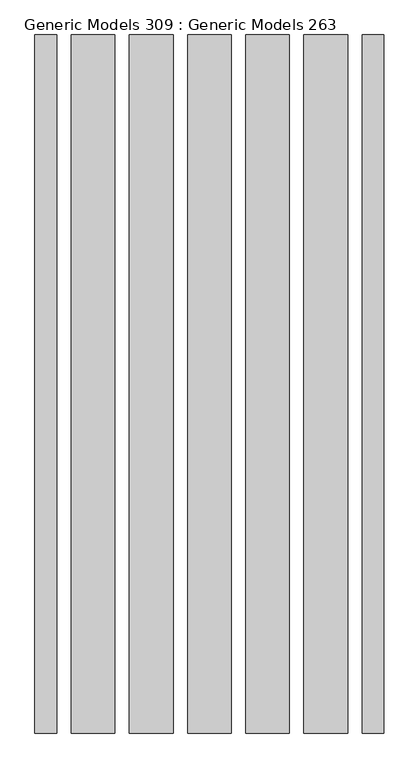
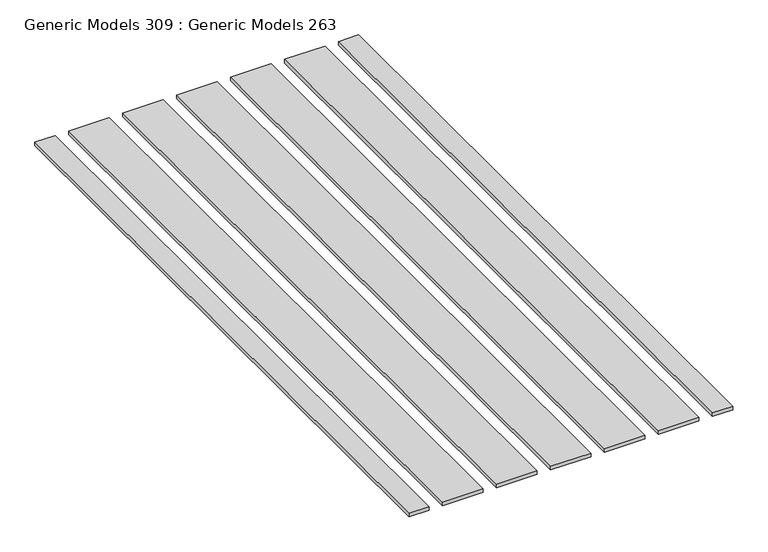
"""IFC4 building model written with IfcOpenShell, lengths in millimetres: proxy geometry, Generic Models 309 : Generic Models 263."""

import ifcopenshell
import ifcopenshell.guid

model = None  # the IFC model being written
_history = None  # IfcOwnerHistory: only IFC2X3 demands one
_inside = {}  # id of a spatial element -> (the spatial element, [elements in it])
_under = {}  # id of a project, library or spatial element -> (it, [spatial elements below it])
_declared = {}  # id of a project -> (the project, [libraries it declares])
_typed = {}  # id of a type object -> (the type object, [elements of that type])
_made_of = {}  # id of a material, layer set ... -> (it, [elements and type objects made of it])


def new_model(schema):
    """Start an empty IFC model of exactly this schema.

    Asked for "IFC4X3", IfcOpenShell would pick the latest addendum, in which some entities
    have other attributes; the version numbers below select the first issue.
    IFC2X3 requires an IfcOwnerHistory on every rooted entity: one is made here for all.
    """
    global model, _history
    if schema == "IFC4X3":
        model = ifcopenshell.file(schema_version=(4, 3, 0, 0))
    else:
        model = ifcopenshell.file(schema=schema)
    _inside.clear()
    _under.clear()
    _declared.clear()
    _typed.clear()
    _made_of.clear()
    _history = None
    if model.schema == "IFC2X3":
        org = make("IfcOrganization", Name="unknown")
        user = make(
            "IfcPersonAndOrganization",
            ThePerson=make("IfcPerson", FamilyName="unknown"),
            TheOrganization=org,
        )
        app = make(
            "IfcApplication",
            ApplicationDeveloper=org,
            Version="unknown",
            ApplicationFullName="unknown",
            ApplicationIdentifier="unknown",
        )
        _history = make(
            "IfcOwnerHistory",
            OwningUser=user,
            OwningApplication=app,
            ChangeAction="ADDED",
            CreationDate=0,
        )
    return model


def make(cls, **values):
    """One entity of the class cls with the attributes given. An attribute that is None is left unset."""
    return model.create_entity(
        cls, **{name: value for name, value in values.items() if value is not None}
    )


def rooted(cls, **values):
    """An entity with a GlobalId (a new one), such as an element, a storey or a relation."""
    return make(cls, GlobalId=ifcopenshell.guid.new(), OwnerHistory=_history, **values)


def si_unit(unit_type, name, prefix=None):
    """IfcSIUnit, for example si_unit("LENGTHUNIT", "METRE", prefix="MILLI")."""
    return make("IfcSIUnit", UnitType=unit_type, Prefix=prefix, Name=name)


def assignment(units):
    """IfcUnitAssignment: the units of a project."""
    return None if units is None else make("IfcUnitAssignment", Units=units)


def point(xyz):
    """IfcCartesianPoint."""
    return None if xyz is None else make("IfcCartesianPoint", Coordinates=xyz)


def direction(xyz):
    """IfcDirection."""
    return None if xyz is None else make("IfcDirection", DirectionRatios=xyz)


def frame(location, z_axis=None, x_axis=None):
    """IfcAxis2Placement3D, a coordinate frame: its origin and axes. An axis left out is left unset."""
    return make(
        "IfcAxis2Placement3D",
        Location=point(location),
        Axis=direction(z_axis),
        RefDirection=direction(x_axis),
    )


def origin():
    """The frame at (0, 0, 0) with its axes left unset."""
    return frame((0.0, 0.0, 0.0))


def place(relative_to, where):
    """IfcLocalPlacement: puts the frame where relative to a parent placement (None: the world)."""
    return make(
        "IfcLocalPlacement", PlacementRelTo=relative_to, RelativePlacement=where
    )


def context(
    kind, dimensions, precision=None, world=None, true_north=None, identifier=None
):
    """IfcGeometricRepresentationContext, for example the 3D "Model" context."""
    return make(
        "IfcGeometricRepresentationContext",
        ContextIdentifier=identifier,
        ContextType=kind,
        CoordinateSpaceDimension=dimensions,
        Precision=precision,
        WorldCoordinateSystem=world,
        TrueNorth=true_north,
    )


def project(units=None, contexts=None):
    """IfcProject with its units and contexts."""
    return rooted(
        "IfcProject",
        Name="project",
        RepresentationContexts=contexts,
        UnitsInContext=assignment(units),
    )


def spatial(cls, under=None, at=None, **own):
    """A site, building, storey or space (cls), placed at a placement, below another one or the project."""
    s = rooted(cls, ObjectPlacement=at, **own)
    if under is not None:
        _under.setdefault(under.id(), (under, []))[1].append(s)
    return s


def polyline(points):
    """IfcPolyline through the points."""
    return make("IfcPolyline", Points=[point(p) for p in points])


def outline(outer, holes=None, kind="AREA"):
    """IfcArbitraryClosedProfileDef: a profile drawn as a closed curve; with holes, ...WithVoids."""
    if holes is None:
        return make("IfcArbitraryClosedProfileDef", ProfileType=kind, OuterCurve=outer)
    return make(
        "IfcArbitraryProfileDefWithVoids",
        ProfileType=kind,
        OuterCurve=outer,
        InnerCurves=holes,
    )


def extrude(swept, where, along, depth):
    """IfcExtrudedAreaSolid: the profile swept, set in the frame where, extruded along a direction by depth."""
    return make(
        "IfcExtrudedAreaSolid",
        SweptArea=swept,
        Position=where,
        ExtrudedDirection=direction(along),
        Depth=depth,
    )


def shape(context_of_items, identifier, shape_type, items):
    """IfcShapeRepresentation: the items that make up one representation, for example the "Body"."""
    return make(
        "IfcShapeRepresentation",
        ContextOfItems=context_of_items,
        RepresentationIdentifier=identifier,
        RepresentationType=shape_type,
        Items=items,
    )


def source(mapping_origin, context_of_items, identifier, shape_type, items):
    """IfcRepresentationMap: a shape defined once, which mapped items show again and again."""
    return make(
        "IfcRepresentationMap",
        MappingOrigin=mapping_origin,
        MappedRepresentation=shape(context_of_items, identifier, shape_type, items),
    )


def transform(
    local_origin,
    x_axis=None,
    y_axis=None,
    z_axis=None,
    scale=None,
    scale2=None,
    scale3=None,
    uniform=True,
):
    """IfcCartesianTransformationOperator3D, or its non-uniform kind. x_axis, y_axis, z_axis: its Axis1, 2, 3."""
    if uniform:
        return make(
            "IfcCartesianTransformationOperator3D",
            Axis1=direction(x_axis),
            Axis2=direction(y_axis),
            LocalOrigin=point(local_origin),
            Scale=scale,
            Axis3=direction(z_axis),
        )
    return make(
        "IfcCartesianTransformationOperator3DnonUniform",
        Axis1=direction(x_axis),
        Axis2=direction(y_axis),
        LocalOrigin=point(local_origin),
        Scale=scale,
        Axis3=direction(z_axis),
        Scale2=scale2,
        Scale3=scale3,
    )


def mapped(mapping_source, mapping_target):
    """IfcMappedItem: shows the shape of a source again, moved by a transform."""
    return make(
        "IfcMappedItem", MappingSource=mapping_source, MappingTarget=mapping_target
    )


def made_of(thing, what):
    """Note that an element or type object is made of a material, layer set ...; save() writes the relation."""
    if what is not None:
        _made_of.setdefault(what.id(), (what, []))[1].append(thing)
    return thing


def element(
    cls,
    number,
    at=None,
    inside=None,
    cuts=None,
    type_object=None,
    material=None,
    context=None,
    identifier="Body",
    shape_type=None,
    held_by="IfcProductDefinitionShape",
    body=None,
    shapes=None,
    **own,
):
    """One element of the class cls, such as IfcWall. Its Tag is "e" and its number.

    at: its placement. inside: the storey or other place that contains it. cuts: it is an
    opening in that element (IfcRelVoidsElement). A single representation is given by context,
    identifier, shape_type and body (its items); several are given by shapes. held_by: the class
    of the entity that holds the representations. save() writes the other relations.
    """
    e = rooted(cls, Tag="e%d" % number, ObjectPlacement=at, **own)
    if body is not None:
        shapes = [shape(context, identifier, shape_type, body)]
    if shapes is not None:
        e.Representation = make(held_by, Representations=shapes)
    if inside is not None:
        _inside.setdefault(inside.id(), (inside, []))[1].append(e)
    if cuts is not None:
        rooted(
            "IfcRelVoidsElement", RelatingBuildingElement=cuts, RelatedOpeningElement=e
        )
    if type_object is not None:
        _typed.setdefault(type_object.id(), (type_object, []))[1].append(e)
    return made_of(e, material)


def aggregate(whole, parts):
    """IfcRelAggregates: a whole, such as a stair, and the parts it consists of."""
    return rooted("IfcRelAggregates", RelatingObject=whole, RelatedObjects=parts)


def save(model, path):
    """Write the relations noted so far, then the file.

    IfcRelAggregates (storeys below a building ...), IfcRelContainedInSpatialStructure (elements
    in a storey), IfcRelDefinesByType, IfcRelAssociatesMaterial and IfcRelDeclares: one each for
    every whole, place, type object, material and project.
    """
    for whole, parts in _under.values():
        aggregate(whole, parts)
    for where, things in _inside.values():
        rooted(
            "IfcRelContainedInSpatialStructure",
            RelatedElements=things,
            RelatingStructure=where,
        )
    for kind, things in _typed.values():
        rooted("IfcRelDefinesByType", RelatedObjects=things, RelatingType=kind)
    for what, things in _made_of.values():
        rooted("IfcRelAssociatesMaterial", RelatedObjects=things, RelatingMaterial=what)
    for by, libraries in _declared.values():
        rooted("IfcRelDeclares", RelatingContext=by, RelatedDefinitions=libraries)
    model.write(path)


def generic_models_309_generic_models_263_71f93402(model_context):
    return source(origin(), model_context, "Body", "SweptSolid", [
        extrude(outline(polyline([(94945.4797726, -94.4486541), (94907.3797726, -94.4486541), (94907.3797726, 1124.7513459), (94945.4797726, 1124.7513459), (94945.4797726, -94.4486541)])), frame((0.0, 0.0, -114.3), z_axis=(0.0, 0.0, 1.0), x_axis=(1.0, 0.0, 0.0)), (0.0, 0.0, 1.0), 7.0017153),
        extrude(outline(polyline([(95516.9797726, -94.4486541), (95478.8797726, -94.4486541), (95478.8797726, 1124.7513459), (95516.9797726, 1124.7513459), (95516.9797726, -94.4486541)])), frame((0.0, 0.0, -114.3), z_axis=(0.0, 0.0, 1.0), x_axis=(1.0, 0.0, 0.0)), (0.0, 0.0, 1.0), 7.0017153),
        extrude(outline(polyline([(95047.0797726, -94.4486541), (94970.8797726, -94.4486541), (94970.8797726, 1124.7513459), (95047.0797726, 1124.7513459), (95047.0797726, -94.4486541)])), frame((0.0, 0.0, -114.3), z_axis=(0.0, 0.0, 1.0), x_axis=(1.0, 0.0, 0.0)), (0.0, 0.0, 1.0), 7.0017153),
        extrude(outline(polyline([(95148.6797726, -94.4486541), (95072.4797726, -94.4486541), (95072.4797726, 1124.7513459), (95148.6797726, 1124.7513459), (95148.6797726, -94.4486541)])), frame((0.0, 0.0, -114.3), z_axis=(0.0, 0.0, 1.0), x_axis=(1.0, 0.0, 0.0)), (0.0, 0.0, 1.0), 7.0017153),
        extrude(outline(polyline([(95250.2797726, -94.4486541), (95174.0797726, -94.4486541), (95174.0797726, 1124.7513459), (95250.2797726, 1124.7513459), (95250.2797726, -94.4486541)])), frame((0.0, 0.0, -114.3), z_axis=(0.0, 0.0, 1.0), x_axis=(1.0, 0.0, 0.0)), (0.0, 0.0, 1.0), 7.0017153),
        extrude(outline(polyline([(95351.8797726, -94.4486541), (95275.6797726, -94.4486541), (95275.6797726, 1124.7513459), (95351.8797726, 1124.7513459), (95351.8797726, -94.4486541)])), frame((0.0, 0.0, -114.3), z_axis=(0.0, 0.0, 1.0), x_axis=(1.0, 0.0, 0.0)), (0.0, 0.0, 1.0), 7.0017153),
        extrude(outline(polyline([(95453.4797726, -94.4486541), (95377.2797726, -94.4486541), (95377.2797726, 1124.7513459), (95453.4797726, 1124.7513459), (95453.4797726, -94.4486541)])), frame((0.0, 0.0, -114.3), z_axis=(0.0, 0.0, 1.0), x_axis=(1.0, 0.0, 0.0)), (0.0, 0.0, 1.0), 7.0017153),
    ])


if __name__ == "__main__":
    model = new_model("IFC4")
    model_context = context("Model", 3, world=origin())
    ifc_project = project(units=[si_unit("LENGTHUNIT", "METRE", prefix="MILLI")], contexts=[model_context])
    site = spatial("IfcSite", under=ifc_project)
    building = spatial("IfcBuilding", under=site)
    placement = place(None, origin())
    generic_models_309_generic_models_263_shape = generic_models_309_generic_models_263_71f93402(model_context)
    element("IfcBuildingElementProxy", 1, Name="Generic Models 309 : Generic Models 263", ObjectType="Generic Models 309 : Generic Models 263", at=placement, inside=building, context=model_context, shape_type="MappedRepresentation", body=[
        mapped(generic_models_309_generic_models_263_shape, transform((0.0, 0.0, 0.0), x_axis=(1.0, 0.0, 0.0), y_axis=(0.0, 1.0, 0.0), z_axis=(0.0, 0.0, 1.0))),
    ])
    save(model, "model.ifc")

# Revit data of these elements
# Element 1 (IfcBuildingElementProxy, "Generic Models 309 : Generic Models 263")
#   Materials on its faces: "EPOXY COATED 6 X 6 X W2.9 X W2.9, PLACED 3\" ABOVE SLAB BASE"
# Materials
#   "EPOXY COATED 6 X 6 X W2.9 X W2.9, PLACED 3\" ABOVE SLAB BASE": class "Miscellaneous", colour RGB 44 44 44, transparency 0, Cost = 0
